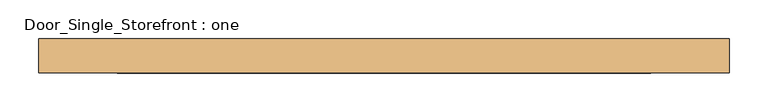
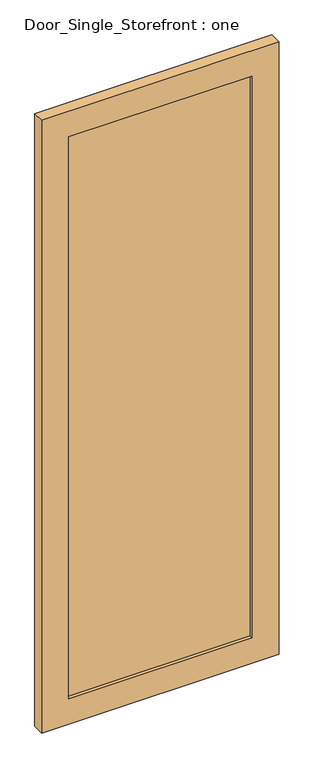
"""IFC4 building model written with IfcOpenShell, lengths in millimetres: door geometry, Door_Single_Storefront : one."""

from ifc_helpers import new_model, si_unit, frame, origin, place, context, project, spatial, polyline, outline, extrude, source, transform, mapped, element, save


def door_single_storefront_one_0563a783(model_context):
    return source(origin(), model_context, "Body", "SweptSolid", [
        extrude(outline(polyline([(345.28125, 6.35), (345.28125, -12.7), (-345.28125, -12.7), (-345.28125, 6.35), (345.28125, 6.35)])), frame((0.0, 0.0, 101.6), z_axis=(0.0, 0.0, 1.0), x_axis=(1.0, 0.0, 0.0)), (0.0, 0.0, 1.0), 2235.2),
        extrude(outline(polyline([(2438.4, -446.88125), (0.0, -446.88125), (0.0, 446.88125), (2438.4, 446.88125), (2438.4, -446.88125)]), holes=[polyline([(101.6, 345.28125), (101.6, -345.28125), (2336.8, -345.28125), (2336.8, 345.28125), (101.6, 345.28125)])]), frame((0.0, -25.4, 0.0), z_axis=(0.0, 1.0, 0.0), x_axis=(0.0, 0.0, 1.0)), (0.0, 0.0, 1.0), 44.45),
    ])


if __name__ == "__main__":
    model = new_model("IFC4")
    model_context = context("Model", 3, world=origin())
    ifc_project = project(units=[si_unit("LENGTHUNIT", "METRE", prefix="MILLI")], contexts=[model_context])
    site = spatial("IfcSite", under=ifc_project)
    building = spatial("IfcBuilding", under=site)
    placement = place(None, origin())
    door_single_storefront_one_shape = door_single_storefront_one_0563a783(model_context)
    element("IfcDoor", 1, ObjectType="Door_Single_Storefront : one", at=placement, inside=building, context=model_context, shape_type="MappedRepresentation", body=[
        mapped(door_single_storefront_one_shape, transform((0.0, 0.0, 0.0), x_axis=(1.0, 0.0, 0.0), y_axis=(0.0, 1.0, 0.0), z_axis=(0.0, 0.0, 1.0))),
    ])
    save(model, "model.ifc")

# Revit data of these elements
# Project information
#   Project Issue Date = "05/21/2015"
#   Project Status = "Project Status"
#   Client Name = "Xcel"
#   Project Address = "Enter address here"
#   Project Name = "Sports Complex"
#   Project Number = "Project Number"
# Type "Door_Single_Storefront : one"
#   Type Mark = "27"
#   Analytic Construction = "<None>"
#   Stile_Width = 0' - 4"
#   Door_Thickness = 0' - 1 3/4"
#   Door_Offset = 0' - 1"
#   Glass_Material = Glass
#   Frame_Material = Aluminum
#   Function = (empty or 0)
# Element 1 (IfcDoor, "Door_Single_Storefront : one")
#   Materials on its faces: "Aluminum", "Glass"
# Materials
#   "Glass": class "Glass", colour RGB 142 168 196, transparency 0.75, Description = "Soda Lime Glass", Cost = 0
#   "Aluminum": class "Metal", colour RGB 226 226 226, transparency 0, Description = "Aluminum 6061", Cost = 0
